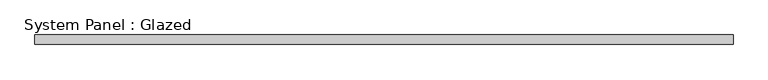
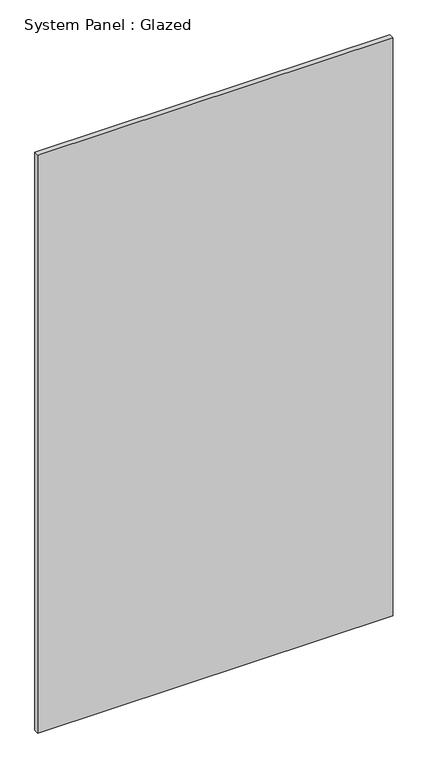
"""IFC4 building model written with IfcOpenShell, lengths in millimetres: plate geometry, System Panel : Glazed."""

from ifc_helpers import new_model, si_unit, origin, origin_with_axes, place, context, project, spatial, polyline, outline, extrude, source, transform, mapped, element, save


def system_panel_glazed_7daaf864(model_context):
    return source(origin(), model_context, "Body", "SweptSolid", [
        extrude(outline(polyline([(920.8333332, 24.5), (-920.8333332, 24.5), (-920.8333332, 49.5), (920.8333332, 49.5), (920.8333332, 24.5)])), origin_with_axes(), (0.0, 0.0, 1.0), 3170.0),
    ])


if __name__ == "__main__":
    model = new_model("IFC4")
    model_context = context("Model", 3, world=origin())
    ifc_project = project(units=[si_unit("LENGTHUNIT", "METRE", prefix="MILLI")], contexts=[model_context])
    site = spatial("IfcSite", under=ifc_project)
    building = spatial("IfcBuilding", under=site)
    placement = place(None, origin())
    system_panel_glazed_shape = system_panel_glazed_7daaf864(model_context)
    element("IfcPlate", 1, ObjectType="System Panel : Glazed", at=placement, inside=building, context=model_context, shape_type="MappedRepresentation", body=[
        mapped(system_panel_glazed_shape, transform((0.0, 0.0, 0.0), x_axis=(1.0, 0.0, 0.0), y_axis=(0.0, 1.0, 0.0), z_axis=(0.0, 0.0, 1.0))),
    ])
    save(model, "model.ifc")

# Revit data of these elements
# Type "System Panel : Glazed"
#   Construction Type Id = "GSP4R"
#   Analytic Construction = "1/8 in Pilkington single glazing"
#   Visual Light Transmittance = 0.9
#   Solar Heat Gain Coefficient = 0.86
#   Heat Transfer Coefficient (U) = 6.7069 W/(m²·K)
#   Define Thermal Properties by = 1
# Element 1 (IfcPlate, "System Panel : Glazed")
#   Materials on its faces: "Glass"
# Materials
#   "Glass": class "Glass", colour RGB 245 245 243, transparency 1, Description = "Soda Lime Glass", Cost = 0
